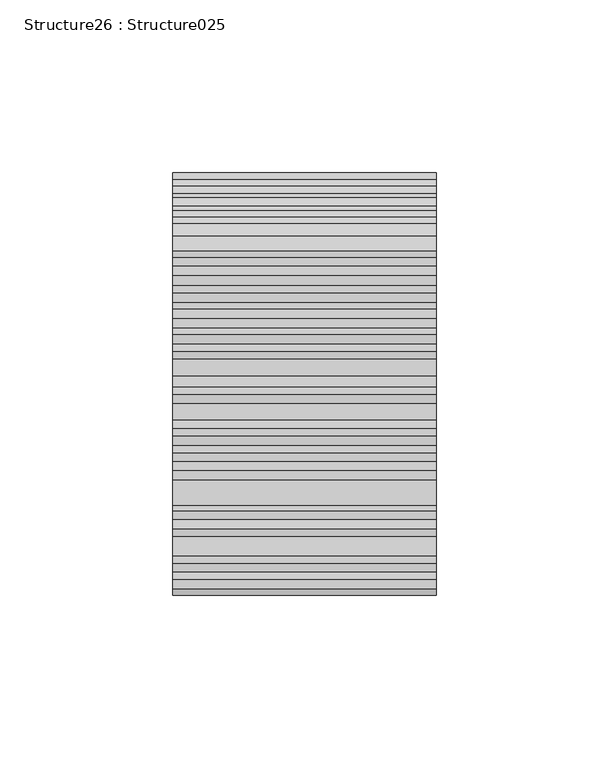
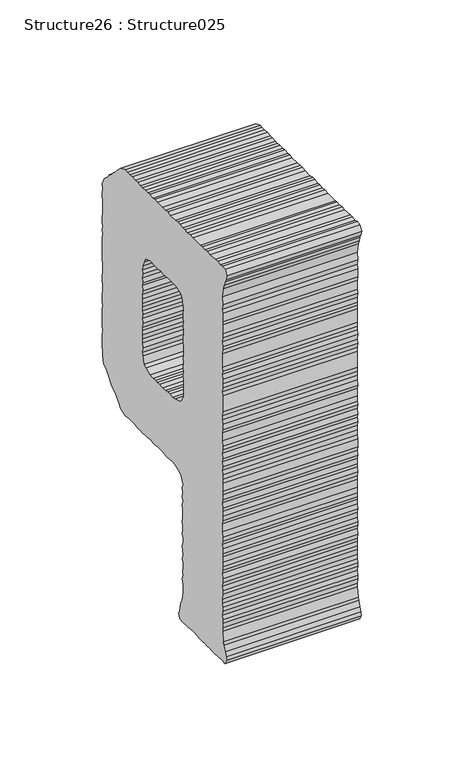
"""IFC4 building model written with IfcOpenShell, lengths in millimetres: proxy geometry, Structure26 : Structure025."""

from ifc_helpers import new_model, si_unit, frame, origin, place, context, project, spatial, polyline, outline, extrude, source, transform, mapped, element, save


def structure26_structure025_f0cf9de2(model_context):
    return source(origin(), model_context, "Body", "SweptSolid", [
        extrude(outline(polyline([(4.6476318, 0.0), (7.4246892, 0.6116643), (9.5892352, 0.3032906), (12.6839852, 0.0), (17.6374491, 0.0), (19.8028423, 0.6116643), (21.9673882, 0.0), (24.7563062, 0.6116643), (26.6040067, 0.3032906), (29.3920774, 0.3032906), (32.1809954, 0.0), (34.0286958, 0.0), (36.8167666, 0.3032906), (38.9821597, 0.3032906), (41.7702305, 0.6116643), (44.5472879, 0.3032906), (47.0185132, 0.3032906), (48.877227, 0.6116643), (53.2071661, -1.2495911), (56.925441, -4.6518676), (58.7731415, -6.8164136), (60.6437158, -8.3565876), (61.879752, -9.9103165), (64.3501301, -11.7571698), (65.5861664, -13.6285913), (67.7507123, -15.7787352), (69.6102734, -17.3324641), (71.4571267, -21.3591126), (70.8454624, -24.1353229), (71.4571267, -26.9115331), (71.4571267, -28.7821075), (70.8454624, -31.5574705), (70.8454624, -38.6780219), (71.4571267, -41.1509415), (71.4571267, -44.2439973), (70.8454624, -46.4220981), (71.1512945, -48.5730892), (70.8454624, -51.046856), (71.1512945, -54.1526194), (71.4571267, -56.3180126), (71.4571267, -58.7773773), (71.1512945, -61.2587687), (71.4571267, -64.3518244), (71.1512945, -66.8255913), (70.8454624, -68.9994562), (70.8454624, -73.9546145), (71.4571267, -76.4122849), (71.4571267, -79.20205), (70.8454624, -81.6851358), (70.8454624, -83.5319891), (71.4571267, -89.1072834), (71.1512945, -91.8885767), (70.8454624, -93.7455962), (71.4571267, -96.8386519), (71.1512945, -98.9947261), (71.4571267, -101.4761175), (71.4571267, -103.9490371), (71.1512945, -106.1144303), (70.8454624, -108.8991123), (71.1512945, -111.6897246), (71.4571267, -114.1617971), (71.4571267, -118.4917362), (70.8454624, -120.9739748), (70.8454624, -123.4418113), (69.9161055, -128.3876506), (67.4448802, -129.6330058), (66.2096912, -131.4807063), (62.4914163, -135.8097982), (60.9376874, -137.3635271), (58.4673093, -138.6004105), (55.3725593, -142.3051305), (53.2071661, -144.7865219), (48.877227, -146.3309318), (47.0185132, -146.0234054), (44.2414558, -145.7057127), (38.9821597, -145.7057127), (36.5109345, -146.3309318), (34.0286958, -146.0234054), (31.5574706, -146.3309318), (29.6979096, -146.0234054), (26.6040067, -146.0234054), (24.4386135, -145.7057127), (21.6615561, -146.3309318), (19.8028423, -146.0234054), (16.7080922, -145.7057127), (12.072321, -145.7057127), (9.283403, -146.3309318), (7.1188571, -146.0234054), (4.9534639, -146.0234054), (2.4822387, -145.7057127), (-0.6235247, -146.3309318), (-4.6357712, -147.5627322), (-5.8718074, -149.1164611), (-7.7305213, -153.1431096), (-7.1069965, -155.3076555), (-7.4246891, -158.3913923), (-7.1069965, -160.8736309), (-7.7305213, -163.0381768), (-7.1069965, -165.20357), (-7.4246891, -168.2966257), (-7.4246891, -172.9434103), (-7.1069965, -175.4163299), (-7.4246891, -177.8892496), (-7.4246891, -180.3570861), (-7.1069965, -183.1468512), (-7.7305213, -185.0038707), (-7.7305213, -187.7843168), (-7.1069965, -190.2530006), (-7.4246891, -193.0520847), (-7.7305213, -195.2073116), (-7.1069965, -197.9970768), (-7.7305213, -199.8540962), (-7.7305213, -202.3270159), (-7.4246891, -205.4065167), (-7.7305213, -207.277091), (-7.1069965, -209.7500107), (-7.7305213, -212.8430664), (-7.7305213, -217.4813792), (-7.1069965, -222.4356902), (-5.5659753, -225.5151911), (-4.6357712, -230.4703493), (-3.4005822, -232.3316047), (-4.6357712, -234.7994412), (-7.1069965, -235.4246604), (-12.378153, -235.4246604), (-15.1552104, -235.1171339), (-17.3206036, -234.7994412), (-19.1793174, -234.7994412), (-24.7444456, -235.4246604), (-26.9098387, -235.4246604), (-29.381064, -235.1171339), (-31.54561, -235.4246604), (-34.0286958, -235.1171339), (-36.8057532, -235.4246604), (-39.2879918, -235.4246604), (-41.1356923, -235.1171339), (-46.3949883, -235.1171339), (-48.5603815, -235.4246604), (-50.4190953, -232.3316047), (-49.807431, -230.4703493), (-48.8780741, -228.0016656), (-47.6420379, -224.9035268), (-47.3243452, -223.0473545), (-46.3949883, -217.4813792), (-46.3949883, -215.315986), (-46.712681, -212.5397758), (-46.712681, -210.3616749), (-46.0891562, -207.8929912), (-46.712681, -205.1125451), (-46.712681, -202.9386801), (-46.0891562, -200.782606), (-46.0891562, -198.3012145), (-46.3949883, -195.2073116), (-46.3949883, -193.0520847), (-46.0891562, -190.569846), (-46.3949883, -188.4053001), (-46.712681, -185.9230614), (-46.0891562, -182.8300057), (-46.712681, -180.6739316), (-46.712681, -178.5000666), (-46.3949883, -176.027147), (-46.3949883, -172.9434103), (-46.712681, -170.7695453), (-46.3949883, -167.9933351), (-46.0891562, -165.5204155), (-46.3949883, -163.663396), (-46.3949883, -161.1904764), (-46.0891562, -158.0838658), (-46.0891562, -153.4464002), (-46.3949883, -151.281007), (-46.712681, -148.496325), (-46.3949883, -145.7057127), (-46.3949883, -143.8580122), (-46.0891562, -140.7649565), (-46.712681, -138.6004105), (-46.3949883, -135.8097982), (-46.712681, -133.6588072), (-46.712681, -128.7044961), (-46.3949883, -126.5255481), (-46.3949883, -123.7493378), (-46.0891562, -121.2772654), (-46.712681, -118.7950268), (-46.0891562, -116.326343), (-46.712681, -114.1617971), (-46.0891562, -111.0645055), (-46.712681, -108.5958217), (-46.3949883, -106.7345663), (-46.0891562, -103.6415106), (-46.0891562, -98.9947261), (-46.712681, -96.8386519), (-46.3949883, -93.7455962), (-46.0891562, -91.2625104), (-46.0891562, -88.7904379), (-46.3949883, -86.3217542), (-46.3949883, -76.7299775), (-46.0891562, -74.5561126), (-46.712681, -71.7756664), (-46.3949883, -69.6102733), (-46.712681, -66.5172176), (-46.0891562, -64.049381), (-46.3949883, -61.8848351), (-46.0891562, -59.715206), (-46.0891562, -51.6669921), (-46.3949883, -49.1983083), (-46.3949883, -47.3362058), (-46.0891562, -44.5515237), (-46.712681, -41.7710776), (-46.3949883, -39.6056845), (-46.3949883, -34.3472356), (-46.712681, -32.1835368), (-46.712681, -27.2292258), (-46.0891562, -25.0638326), (-46.712681, -21.9843318), (-46.0891562, -17.6408378), (-47.3243452, -12.0748625), (-48.2537021, -9.6019428), (-48.8780741, -7.1332591), (-49.807431, -5.2720037), (-50.7249274, -2.4864745), (-48.8780741, 0.3032906), (-46.0891562, 0.6116643), (-43.923763, 0.0), (-41.4533849, 0.6116643), (-39.2879918, 0.6116643), (-33.7228636, 0.0), (-31.54561, 0.6116643), (-28.7685526, 0.0), (-26.2981745, 0.3032906), (-24.7444456, 0.0), (-17.3206036, 0.0), (-14.5435462, 0.3032906), (-12.0604604, 0.0), (-9.5900823, 0.3032906), (-7.4246891, 0.0), (-4.6357712, 0.6116643), (-2.4712252, 0.6116643), (0.0, 0.0), (4.6476318, 0.0)]), holes=[polyline([(-4.9416033, -105.1943923), (0.0, -106.7345663), (2.164546, -107.04294), (4.9534639, -106.7345663), (7.4246892, -107.04294), (9.283403, -107.04294), (12.072321, -107.3453834), (14.8493784, -107.04294), (17.3197565, -107.3453834), (19.1793175, -107.04294), (21.6615561, -107.3453834), (24.4386135, -107.04294), (28.1568884, -105.1943923), (30.3222815, -104.2658826), (31.2397779, -99.9367907), (31.8633027, -98.0755353), (31.2397779, -94.9824796), (31.8633027, -92.5087128), (31.8633027, -90.040029), (31.5574706, -87.5544017), (31.8633027, -85.085718), (31.5574706, -82.9076171), (31.2397779, -80.4389334), (31.8633027, -77.9668609), (31.2397779, -75.1770958), (31.8633027, -73.3285481), (31.5574706, -70.8471567), (31.5574706, -68.6817636), (31.8633027, -66.2130798), (31.8633027, -63.4233147), (31.2397779, -60.9512423), (31.8633027, -58.1741848), (31.2397779, -56.3180126), (31.5574706, -53.5282474), (31.2397779, -50.7384823), (31.5574706, -48.5730892), (31.2397779, -46.1060998), (29.6979096, -42.7038233), (28.7804132, -40.8425679), (24.7563062, -39.2896862), (19.8028423, -39.2896862), (16.7080922, -39.6056845), (14.5435463, -38.9855484), (11.7546283, -39.6056845), (9.9069278, -39.2896862), (7.4246892, -38.9855484), (-0.3058321, -38.9855484), (-4.9416033, -40.5392773), (-6.4953322, -42.3954496), (-7.4246891, -46.1060998), (-7.7305213, -48.5730892), (-7.4246891, -51.046856), (-7.4246891, -53.8459401), (-8.0363534, -56.3180126), (-7.4246891, -58.1741848), (-7.7305213, -61.2587687), (-8.0363534, -63.4233147), (-7.4246891, -65.9064005), (-7.4246891, -68.0709465), (-7.7305213, -70.529464), (-7.7305213, -75.4837751), (-7.4246891, -78.2837064), (-7.7305213, -80.1322541), (-7.4246891, -82.9076171), (-7.7305213, -85.7117843), (-7.4246891, -87.8627754), (-8.0363534, -90.6381384), (-7.7305213, -92.5087128), (-8.0363534, -94.9824796), (-7.7305213, -98.0755353), (-7.7305213, -100.5476078), (-6.1895001, -103.9490371), (-4.9416033, -105.1943923)])]), frame((-35624.0862846, 276457.8424197, 4217.9376236), z_axis=(1.0, 0.0, 1.354250045437766e-12), x_axis=(0.0, 1.0, 0.0)), (0.0, 0.0, 1.0), 76.2),
    ])


if __name__ == "__main__":
    model = new_model("IFC4")
    model_context = context("Model", 3, world=origin())
    ifc_project = project(units=[si_unit("LENGTHUNIT", "METRE", prefix="MILLI")], contexts=[model_context])
    site = spatial("IfcSite", under=ifc_project)
    building = spatial("IfcBuilding", under=site)
    placement = place(None, origin())
    structure26_structure025_shape = structure26_structure025_f0cf9de2(model_context)
    element("IfcBuildingElementProxy", 1, Name="Structure26 : Structure025", ObjectType="Structure26 : Structure025", at=placement, inside=building, context=model_context, shape_type="MappedRepresentation", body=[
        mapped(structure26_structure025_shape, transform((0.0, 0.0, 0.0), x_axis=(1.0, 0.0, 0.0), y_axis=(0.0, 1.0, 0.0), z_axis=(0.0, 0.0, 1.0))),
    ])
    save(model, "model.ifc")

# Revit data of these elements
# Type "Structure26 : Structure025"
#   NameOverride = "Structure025"
# Element 1 (IfcBuildingElementProxy, "Structure26 : Structure025")
#   Materials on its faces: "BRUSHED ALUMINUM LETTERING"
# Materials
#   "BRUSHED ALUMINUM LETTERING": class "Unassigned", colour RGB 169 181 186, transparency 0, Cost = 0
